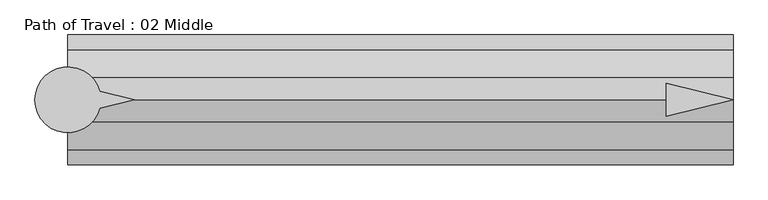
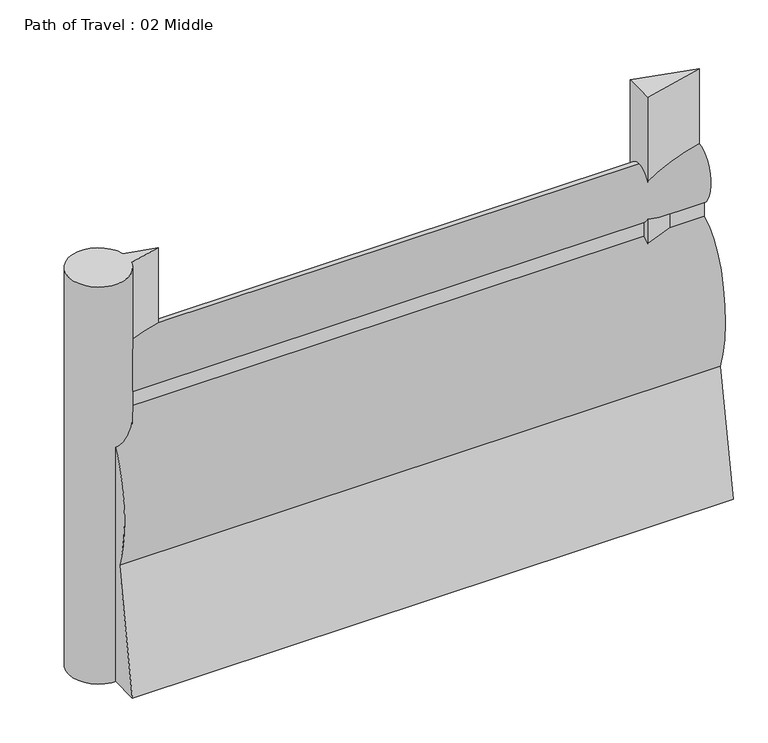
"""IFC4 building model written with IfcOpenShell, lengths in millimetres: proxy geometry, Path of Travel : 02 Middle."""

import ifcopenshell
import ifcopenshell.guid

model = None  # the IFC model being written
_history = None  # IfcOwnerHistory: only IFC2X3 demands one
_inside = {}  # id of a spatial element -> (the spatial element, [elements in it])
_under = {}  # id of a project, library or spatial element -> (it, [spatial elements below it])
_declared = {}  # id of a project -> (the project, [libraries it declares])
_typed = {}  # id of a type object -> (the type object, [elements of that type])
_made_of = {}  # id of a material, layer set ... -> (it, [elements and type objects made of it])


def new_model(schema):
    """Start an empty IFC model of exactly this schema.

    Asked for "IFC4X3", IfcOpenShell would pick the latest addendum, in which some entities
    have other attributes; the version numbers below select the first issue.
    IFC2X3 requires an IfcOwnerHistory on every rooted entity: one is made here for all.
    """
    global model, _history
    if schema == "IFC4X3":
        model = ifcopenshell.file(schema_version=(4, 3, 0, 0))
    else:
        model = ifcopenshell.file(schema=schema)
    _inside.clear()
    _under.clear()
    _declared.clear()
    _typed.clear()
    _made_of.clear()
    _history = None
    if model.schema == "IFC2X3":
        org = make("IfcOrganization", Name="unknown")
        user = make(
            "IfcPersonAndOrganization",
            ThePerson=make("IfcPerson", FamilyName="unknown"),
            TheOrganization=org,
        )
        app = make(
            "IfcApplication",
            ApplicationDeveloper=org,
            Version="unknown",
            ApplicationFullName="unknown",
            ApplicationIdentifier="unknown",
        )
        _history = make(
            "IfcOwnerHistory",
            OwningUser=user,
            OwningApplication=app,
            ChangeAction="ADDED",
            CreationDate=0,
        )
    return model


def make(cls, **values):
    """One entity of the class cls with the attributes given. An attribute that is None is left unset."""
    return model.create_entity(
        cls, **{name: value for name, value in values.items() if value is not None}
    )


def rooted(cls, **values):
    """An entity with a GlobalId (a new one), such as an element, a storey or a relation."""
    return make(cls, GlobalId=ifcopenshell.guid.new(), OwnerHistory=_history, **values)


def si_unit(unit_type, name, prefix=None):
    """IfcSIUnit, for example si_unit("LENGTHUNIT", "METRE", prefix="MILLI")."""
    return make("IfcSIUnit", UnitType=unit_type, Prefix=prefix, Name=name)


def assignment(units):
    """IfcUnitAssignment: the units of a project."""
    return None if units is None else make("IfcUnitAssignment", Units=units)


def point(xyz):
    """IfcCartesianPoint."""
    return None if xyz is None else make("IfcCartesianPoint", Coordinates=xyz)


def direction(xyz):
    """IfcDirection."""
    return None if xyz is None else make("IfcDirection", DirectionRatios=xyz)


def frame(location, z_axis=None, x_axis=None):
    """IfcAxis2Placement3D, a coordinate frame: its origin and axes. An axis left out is left unset."""
    return make(
        "IfcAxis2Placement3D",
        Location=point(location),
        Axis=direction(z_axis),
        RefDirection=direction(x_axis),
    )


def frame_2d(location, x_axis=None):
    """IfcAxis2Placement2D, a coordinate frame in the plane: its origin and x axis."""
    return make(
        "IfcAxis2Placement2D", Location=point(location), RefDirection=direction(x_axis)
    )


def origin():
    """The frame at (0, 0, 0) with its axes left unset."""
    return frame((0.0, 0.0, 0.0))


def origin_with_axes():
    """The frame at (0, 0, 0) with the z axis (0, 0, 1) and the x axis (1, 0, 0) written out."""
    return frame((0.0, 0.0, 0.0), z_axis=(0.0, 0.0, 1.0), x_axis=(1.0, 0.0, 0.0))


def place(relative_to, where):
    """IfcLocalPlacement: puts the frame where relative to a parent placement (None: the world)."""
    return make(
        "IfcLocalPlacement", PlacementRelTo=relative_to, RelativePlacement=where
    )


def context(
    kind, dimensions, precision=None, world=None, true_north=None, identifier=None
):
    """IfcGeometricRepresentationContext, for example the 3D "Model" context."""
    return make(
        "IfcGeometricRepresentationContext",
        ContextIdentifier=identifier,
        ContextType=kind,
        CoordinateSpaceDimension=dimensions,
        Precision=precision,
        WorldCoordinateSystem=world,
        TrueNorth=true_north,
    )


def project(units=None, contexts=None):
    """IfcProject with its units and contexts."""
    return rooted(
        "IfcProject",
        Name="project",
        RepresentationContexts=contexts,
        UnitsInContext=assignment(units),
    )


def spatial(cls, under=None, at=None, **own):
    """A site, building, storey or space (cls), placed at a placement, below another one or the project."""
    s = rooted(cls, ObjectPlacement=at, **own)
    if under is not None:
        _under.setdefault(under.id(), (under, []))[1].append(s)
    return s


def polyline(points):
    """IfcPolyline through the points."""
    return make("IfcPolyline", Points=[point(p) for p in points])


def circle_curve(where, radius):
    """IfcCircle in the frame where."""
    return make("IfcCircle", Position=where, Radius=radius)


def ellipse_curve(where, semi_axis1, semi_axis2):
    """IfcEllipse in the frame where."""
    return make(
        "IfcEllipse", Position=where, SemiAxis1=semi_axis1, SemiAxis2=semi_axis2
    )


def trimmed(basis, trim1, trim2, sense, master):
    """IfcTrimmedCurve: the piece of a basis curve between two trims."""
    return make(
        "IfcTrimmedCurve",
        BasisCurve=basis,
        Trim1=trim1,
        Trim2=trim2,
        SenseAgreement=sense,
        MasterRepresentation=master,
    )


def segment(curve, same_sense, transition):
    """IfcCompositeCurveSegment."""
    return make(
        "IfcCompositeCurveSegment",
        Transition=transition,
        SameSense=same_sense,
        ParentCurve=curve,
    )


def composite_curve(segments, self_intersect=None):
    """IfcCompositeCurve: segments joined end to end."""
    return make("IfcCompositeCurve", Segments=segments, SelfIntersect=self_intersect)


def outline(outer, holes=None, kind="AREA"):
    """IfcArbitraryClosedProfileDef: a profile drawn as a closed curve; with holes, ...WithVoids."""
    if holes is None:
        return make("IfcArbitraryClosedProfileDef", ProfileType=kind, OuterCurve=outer)
    return make(
        "IfcArbitraryProfileDefWithVoids",
        ProfileType=kind,
        OuterCurve=outer,
        InnerCurves=holes,
    )


def extrude(swept, where, along, depth):
    """IfcExtrudedAreaSolid: the profile swept, set in the frame where, extruded along a direction by depth."""
    return make(
        "IfcExtrudedAreaSolid",
        SweptArea=swept,
        Position=where,
        ExtrudedDirection=direction(along),
        Depth=depth,
    )


def shape(context_of_items, identifier, shape_type, items):
    """IfcShapeRepresentation: the items that make up one representation, for example the "Body"."""
    return make(
        "IfcShapeRepresentation",
        ContextOfItems=context_of_items,
        RepresentationIdentifier=identifier,
        RepresentationType=shape_type,
        Items=items,
    )


def source(mapping_origin, context_of_items, identifier, shape_type, items):
    """IfcRepresentationMap: a shape defined once, which mapped items show again and again."""
    return make(
        "IfcRepresentationMap",
        MappingOrigin=mapping_origin,
        MappedRepresentation=shape(context_of_items, identifier, shape_type, items),
    )


def transform(
    local_origin,
    x_axis=None,
    y_axis=None,
    z_axis=None,
    scale=None,
    scale2=None,
    scale3=None,
    uniform=True,
):
    """IfcCartesianTransformationOperator3D, or its non-uniform kind. x_axis, y_axis, z_axis: its Axis1, 2, 3."""
    if uniform:
        return make(
            "IfcCartesianTransformationOperator3D",
            Axis1=direction(x_axis),
            Axis2=direction(y_axis),
            LocalOrigin=point(local_origin),
            Scale=scale,
            Axis3=direction(z_axis),
        )
    return make(
        "IfcCartesianTransformationOperator3DnonUniform",
        Axis1=direction(x_axis),
        Axis2=direction(y_axis),
        LocalOrigin=point(local_origin),
        Scale=scale,
        Axis3=direction(z_axis),
        Scale2=scale2,
        Scale3=scale3,
    )


def mapped(mapping_source, mapping_target):
    """IfcMappedItem: shows the shape of a source again, moved by a transform."""
    return make(
        "IfcMappedItem", MappingSource=mapping_source, MappingTarget=mapping_target
    )


def made_of(thing, what):
    """Note that an element or type object is made of a material, layer set ...; save() writes the relation."""
    if what is not None:
        _made_of.setdefault(what.id(), (what, []))[1].append(thing)
    return thing


def element(
    cls,
    number,
    at=None,
    inside=None,
    cuts=None,
    type_object=None,
    material=None,
    context=None,
    identifier="Body",
    shape_type=None,
    held_by="IfcProductDefinitionShape",
    body=None,
    shapes=None,
    **own,
):
    """One element of the class cls, such as IfcWall. Its Tag is "e" and its number.

    at: its placement. inside: the storey or other place that contains it. cuts: it is an
    opening in that element (IfcRelVoidsElement). A single representation is given by context,
    identifier, shape_type and body (its items); several are given by shapes. held_by: the class
    of the entity that holds the representations. save() writes the other relations.
    """
    e = rooted(cls, Tag="e%d" % number, ObjectPlacement=at, **own)
    if body is not None:
        shapes = [shape(context, identifier, shape_type, body)]
    if shapes is not None:
        e.Representation = make(held_by, Representations=shapes)
    if inside is not None:
        _inside.setdefault(inside.id(), (inside, []))[1].append(e)
    if cuts is not None:
        rooted(
            "IfcRelVoidsElement", RelatingBuildingElement=cuts, RelatedOpeningElement=e
        )
    if type_object is not None:
        _typed.setdefault(type_object.id(), (type_object, []))[1].append(e)
    return made_of(e, material)


def aggregate(whole, parts):
    """IfcRelAggregates: a whole, such as a stair, and the parts it consists of."""
    return rooted("IfcRelAggregates", RelatingObject=whole, RelatedObjects=parts)


def save(model, path):
    """Write the relations noted so far, then the file.

    IfcRelAggregates (storeys below a building ...), IfcRelContainedInSpatialStructure (elements
    in a storey), IfcRelDefinesByType, IfcRelAssociatesMaterial and IfcRelDeclares: one each for
    every whole, place, type object, material and project.
    """
    for whole, parts in _under.values():
        aggregate(whole, parts)
    for where, things in _inside.values():
        rooted(
            "IfcRelContainedInSpatialStructure",
            RelatedElements=things,
            RelatingStructure=where,
        )
    for kind, things in _typed.values():
        rooted("IfcRelDefinesByType", RelatedObjects=things, RelatingType=kind)
    for what, things in _made_of.values():
        rooted("IfcRelAssociatesMaterial", RelatedObjects=things, RelatingMaterial=what)
    for by, libraries in _declared.values():
        rooted("IfcRelDeclares", RelatingContext=by, RelatedDefinitions=libraries)
    model.write(path)


def plane_surface(at):
    """IfcPlane: the flat surface through the origin of the frame at, square to its z axis."""
    return make("IfcPlane", Position=at)


def extruded_surface(curve, direction_of_extrusion, depth):
    """IfcSurfaceOfLinearExtrusion: the curve pushed along a direction by depth."""
    return make(
        "IfcSurfaceOfLinearExtrusion",
        SweptCurve=make("IfcArbitraryOpenProfileDef", ProfileType="CURVE", Curve=curve),
        ExtrudedDirection=direction(direction_of_extrusion),
        Depth=depth,
    )


def advanced_brep(points, edges, surfaces, faces):
    """IfcAdvancedBrep: a solid bounded by faces that lie on surfaces and meet in shared edges.

    An edge is (start, end): straight between two places in points (the first is 0);
    or (start, end, curve); or (start, end, curve, False) where it runs against its curve.
    A face is (place in surfaces, loops), or (place, loops, False) where it looks against
    its surface's normal. A loop lists edges by number (the first is 1), with a minus sign
    where the edge is run from its end to its start. The first loop is the outer one.
    """
    corners = [point(p) for p in points]
    vertices = [make("IfcVertexPoint", VertexGeometry=c) for c in corners]
    made = []
    for start, end, *more in edges:
        made.append(
            make(
                "IfcEdgeCurve",
                EdgeStart=vertices[start],
                EdgeEnd=vertices[end],
                EdgeGeometry=more[0] if more else make("IfcPolyline", Points=[corners[start], corners[end]]),
                SameSense=more[1] if len(more) > 1 else True,
            )
        )
    hull = []
    for where, loops, *sense in faces:
        bounds = []
        for j, loop in enumerate(loops):
            ring = [make("IfcOrientedEdge", EdgeElement=made[abs(k) - 1], Orientation=k > 0) for k in loop]
            bounds.append(
                make(
                    "IfcFaceOuterBound" if j == 0 else "IfcFaceBound",
                    Bound=make("IfcEdgeLoop", EdgeList=ring),
                    Orientation=True,
                )
            )
        hull.append(make("IfcAdvancedFace", Bounds=bounds, FaceSurface=surfaces[where], SameSense=sense[0] if sense else True))
    return make("IfcAdvancedBrep", Outer=make("IfcClosedShell", CfsFaces=hull))


def path_of_travel_02_middle_d5dfa4f0(model_context):
    return source(origin(), model_context, "Body", "SolidModel", [
        advanced_brep(
        [(227.5554837, 0.0, 1727.2), (227.5554837, 42.9018657, 1436.6534209), (227.5554837, 42.9018657, 1363.4763406), (227.5554837, 184.1186263, 643.4144547), (227.5554837, 297.5699544, 0.0), (227.5554837, 145.6574193, 0.0), (227.5554837, 0.0, 584.2), (227.5554837, -145.6574193, 0.0), (227.5554837, -297.5699544, 0.0), (227.5554837, -184.1186263, 643.4144547), (227.5554837, -42.9018657, 1363.4763406), (227.5554837, -42.9018657, 1436.6534209), (3275.5554837, 0.0, 1727.2), (3275.5554837, -42.9018657, 1436.6534209), (3275.5554837, -42.9018657, 1363.4763406), (3275.5554837, -184.1186263, 643.4144547), (3275.5554837, -297.5699544, 0.0), (3275.5554837, -145.6574193, 0.0), (3275.5554837, 0.0, 584.2), (3275.5554837, 145.6574193, 0.0), (3275.5554837, 297.5699544, 0.0), (3275.5554837, 184.1186263, 643.4144547), (3275.5554837, 42.9018657, 1363.4763406), (3275.5554837, 42.9018657, 1436.6534209)],
        [
            (0, 1, ellipse_curve(frame((227.5554837, 0.0, 1574.8), z_axis=(-1.0, 0.0, 0.0), x_axis=(0.0, 0.0, 1.0)), 152.4, 101.6)),
            (1, 2),
            (2, 3, ellipse_curve(frame((227.5554837, 0.0, 914.4), z_axis=(-1.0, 0.0, 0.0), x_axis=(0.0, 0.0, -1.0)), 457.2, 228.6)),
            (3, 4),
            (4, 5),
            (5, 6),
            (6, 7),
            (7, 8),
            (8, 9),
            (9, 10, ellipse_curve(frame((227.5554837, 0.0, 914.4), z_axis=(-1.0, 0.0, 0.0), x_axis=(0.0, 0.0, -1.0)), 457.2, 228.6)),
            (10, 11),
            (11, 0, ellipse_curve(frame((227.5554837, 0.0, 1574.8), z_axis=(-1.0, 0.0, 0.0), x_axis=(0.0, 0.0, 1.0)), 152.4, 101.6)),
            (12, 13, ellipse_curve(frame((3275.5554837, 0.0, 1574.8), z_axis=(1.0, 0.0, 0.0), x_axis=(0.0, 0.0, 1.0)), 152.4, 101.6)),
            (13, 14),
            (14, 15, ellipse_curve(frame((3275.5554837, 0.0, 914.4), z_axis=(1.0, 0.0, 0.0), x_axis=(0.0, 0.0, -1.0)), 457.2, 228.6)),
            (15, 16),
            (16, 17),
            (17, 18),
            (18, 19),
            (19, 20),
            (20, 21),
            (21, 22, ellipse_curve(frame((3275.5554837, 0.0, 914.4), z_axis=(1.0, 0.0, 0.0), x_axis=(0.0, 0.0, -1.0)), 457.2, 228.6)),
            (22, 23),
            (23, 12, ellipse_curve(frame((3275.5554837, 0.0, 1574.8), z_axis=(1.0, 0.0, 0.0), x_axis=(0.0, 0.0, 1.0)), 152.4, 101.6)),
            (0, 12),
            (23, 1),
            (22, 2),
            (21, 3),
            (20, 4),
            (19, 5),
            (18, 6),
            (17, 7),
            (16, 8),
            (15, 9),
            (14, 10),
            (13, 11),
        ],
        [
            plane_surface(frame((227.5554837, 0.0, 0.0), z_axis=(-1.0, 0.0, 0.0), x_axis=(0.0, 0.0, 1.0))),
            plane_surface(frame((3275.5554837, 0.0, 0.0), z_axis=(1.0, 0.0, 0.0), x_axis=(0.0, 0.0, 1.0))),
            extruded_surface(trimmed(ellipse_curve(frame((3275.5554837, 0.0, 1574.8), z_axis=(-1.0, 0.0, 0.0), x_axis=(0.0, 0.0, 1.0)), 152.4, 101.6), [point((3275.5554837, 0.0, 1727.2))], [point((3275.5554837, 42.9018657, 1436.6534209))], True, "CARTESIAN"), (-3048.0, 0.0, 0.0), 3048.0),
            plane_surface(frame((227.5554837, 42.9018657, 1436.6534209), z_axis=(0.0, 1.0, 0.0), x_axis=(1.0, 0.0, 0.0))),
            extruded_surface(trimmed(ellipse_curve(frame((3275.5554837, 0.0, 914.4), z_axis=(-1.0, 0.0, 0.0), x_axis=(0.0, 0.0, -1.0)), 457.2, 228.6), [point((3275.5554837, 42.9018657, 1363.4763406))], [point((3275.5554837, 184.1186263, 643.4144547))], True, "CARTESIAN"), (-3048.0, 0.0, 0.0), 3048.0),
            plane_surface(frame((227.5554837, 184.1186263, 643.4144547), z_axis=(0.0, 0.9848077530122078, 0.1736481776669322), x_axis=(1.0, 0.0, 0.0))),
            plane_surface(frame((227.5554837, 297.5699544, 0.0), z_axis=(0.0, 0.0, -1.0), x_axis=(1.0, 0.0, 0.0))),
            plane_surface(frame((227.5554837, 145.6574193, 0.0), z_axis=(0.0, -0.9702957262760199, -0.2419218955995739), x_axis=(1.0, 0.0, 0.0))),
            plane_surface(frame((227.5554837, 0.0, 584.2), z_axis=(0.0, 0.9702957262759961, -0.24192189559966923), x_axis=(1.0, 0.0, 0.0))),
            plane_surface(frame((227.5554837, -145.6574193, 0.0), z_axis=(0.0, 0.0, -1.0), x_axis=(1.0, 0.0, 0.0))),
            plane_surface(frame((227.5554837, -297.5699544, 0.0), z_axis=(0.0, -0.984807753012208, 0.17364817766693066), x_axis=(1.0, 0.0, 0.0))),
            extruded_surface(trimmed(ellipse_curve(frame((3275.5554837, 0.0, 914.4), z_axis=(-1.0, 0.0, 0.0), x_axis=(0.0, 0.0, -1.0)), 457.2, 228.6), [point((3275.5554837, -184.1186263, 643.4144547))], [point((3275.5554837, -42.9018657, 1363.4763406))], True, "CARTESIAN"), (-3048.0, 0.0, 0.0), 3048.0),
            plane_surface(frame((227.5554837, -42.9018657, 1363.4763406), z_axis=(0.0, -1.0, 0.0), x_axis=(1.0, 0.0, 0.0))),
            extruded_surface(trimmed(ellipse_curve(frame((3275.5554837, 0.0, 1574.8), z_axis=(-1.0, 0.0, 0.0), x_axis=(0.0, 0.0, 1.0)), 152.4, 101.6), [point((3275.5554837, -42.9018657, 1436.6534209))], [point((3275.5554837, 0.0, 1727.2))], True, "CARTESIAN"), (-3048.0, 0.0, 0.0), 3048.0),
        ],
        [
            (0, [[1, 2, 3, 4, 5, 6, 7, 8, 9, 10, 11, 12]]),
            (1, [[13, 14, 15, 16, 17, 18, 19, 20, 21, 22, 23, 24]]),
            (2, [[-1, 25, -24, 26]]),
            (3, [[-2, -26, -23, 27]]),
            (4, [[-3, -27, -22, 28]]),
            (5, [[-4, -28, -21, 29]]),
            (6, [[-5, -29, -20, 30]]),
            (7, [[-6, -30, -19, 31]]),
            (8, [[-7, -31, -18, 32]]),
            (9, [[-8, -32, -17, 33]]),
            (10, [[-9, -33, -16, 34]]),
            (11, [[-10, -34, -15, 35]]),
            (12, [[-11, -35, -14, 36]]),
            (13, [[-12, -36, -13, -25]]),
        ],
    ),
        extrude(outline(polyline([(2969.5503371, 76.2006338), (3275.5554837, 0.0), (2969.5503371, -76.2006338), (2969.5503371, 76.2006338)])), origin_with_axes(), (0.0, 0.0, 1.0), 2129.5973753),
        extrude(outline(composite_curve([segment(polyline([(372.7837828, 39.4440225), (531.182385, 0.0), (372.7837828, -39.4440225)]), True, "CONTINUOUS"), segment(trimmed(circle_curve(frame_2d((227.2200886, 0.0)), 150.8131956), [point((372.7837828, -39.4440225))], [point((372.7837828, 39.4440225))], False, "CARTESIAN"), True, "CONTINUOUS")], self_intersect=False)), origin_with_axes(), (0.0, 0.0, 1.0), 2129.5973753),
    ])


if __name__ == "__main__":
    model = new_model("IFC4")
    model_context = context("Model", 3, world=origin())
    ifc_project = project(units=[si_unit("LENGTHUNIT", "METRE", prefix="MILLI")], contexts=[model_context])
    site = spatial("IfcSite", under=ifc_project)
    building = spatial("IfcBuilding", under=site)
    placement = place(None, origin())
    path_of_travel_02_middle_shape = path_of_travel_02_middle_d5dfa4f0(model_context)
    element("IfcBuildingElementProxy", 1, Name="Path of Travel : 02 Middle", ObjectType="Path of Travel : 02 Middle", at=placement, inside=building, context=model_context, shape_type="MappedRepresentation", body=[
        mapped(path_of_travel_02_middle_shape, transform((0.0, 0.0, 0.0), x_axis=(1.0, 0.0, 0.0), y_axis=(0.0, 1.0, 0.0), z_axis=(0.0, 0.0, 1.0))),
    ])
    save(model, "model.ifc")

# Revit data of these elements
# Type "Path of Travel : 02 Middle"
#   Path of Egress [instance default] = 4' - 0"
#   built-in parameter 1001306 [instance default] = 4 (stored number, unit not read)
#   Dot at Start = no
#   Arrow in Middle = yes
#   Arrow at End = no
#   Egress Path = none
# Element 1 (IfcBuildingElementProxy, "Path of Travel : 02 Middle")
#   Path of Egress = 10' - 0"
#   built-in parameter 1001306 = 10 (stored number, unit not read)
